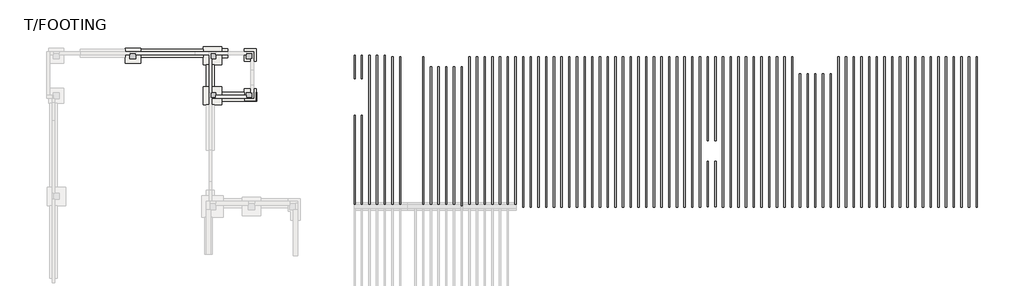
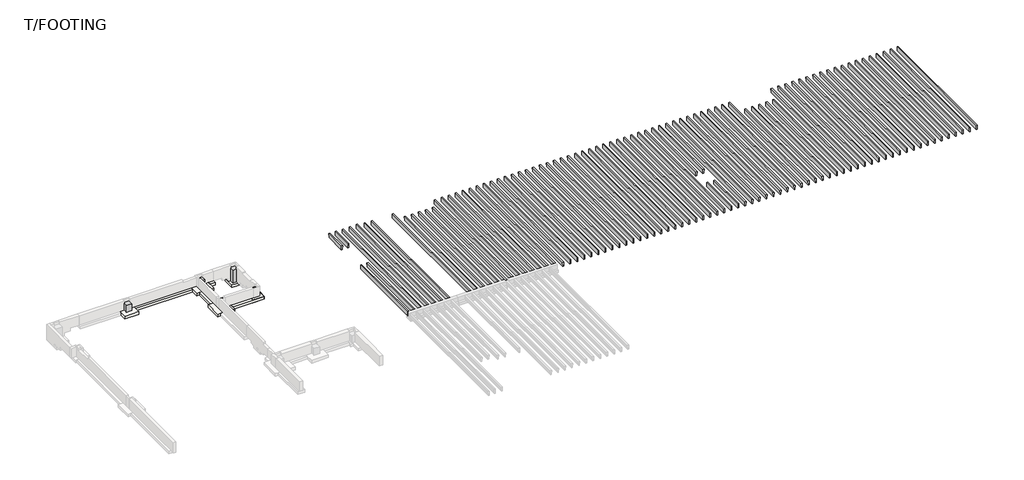
# One storey, part 3 of 3: 84 beams, 5 columns, 5 slabs, 4 footings.
# Revit data of these elements (continued)
# Elements 1, 2, 3, 4, 5, 6, 7, 8, 9, 10, 11, 12, 13, 14, 15, 16, 17, 18, 19, 20, 21, 22, 23, 24, 25, 26, 27, 28, 29, 30, 31, 32, 33, 34, 35, 36, 37, 38, 39, 40, 41, 42, 43, 44, 45, 46, 47, 48, 49, 50, 51, 52, 53, 54, 55, 56, 57, 58, 59, 60, 61, 62, 63, 82, 83, 84 (IfcBeam, "Precast-Cone Shaped Beam : DOUBLE_T") (continued)
#   Materials on its faces: "Concrete - Precast Concrete - Normal Weight Concrete - 5 ksi"
# Elements 64, 65 (IfcBeam, "Precast-Cone Shaped Beam : DOUBLE_T")
#   Comments = ""
#   Tie Rod Weight = 30
#   Tie Rod W = 0.0660938 kip
#   Single Rebar Weight = 50
#   Single Rebar W = 0.110156 kip
#   Rebar Grids Weight = 100
#   Rebar Grids W = 0.220313 kip
#   Length = 27' - 5 11/16"
#   Structural Material = Concrete - Precast Concrete - Normal Weight Concrete - 5 ksi
#   Phase Created = New Construction
#   Materials on its faces: "Concrete - Precast Concrete - Normal Weight Concrete - 5 ksi"
# Elements 66, 67 (IfcBeam, "Precast-Cone Shaped Beam : DOUBLE_T")
#   Comments = ""
#   Tie Rod Weight = 30
#   Tie Rod W = 0.0660938 kip
#   Single Rebar Weight = 50
#   Single Rebar W = 0.110156 kip
#   Rebar Grids Weight = 100
#   Rebar Grids W = 0.220313 kip
#   Length = 14' - 4 11/16"
#   Structural Material = Concrete - Precast Concrete - Normal Weight Concrete - 5 ksi
#   Phase Created = New Construction
#   Materials on its faces: "Concrete - Precast Concrete - Normal Weight Concrete - 5 ksi"
# Elements 68, 69, 70, 71, 72 (IfcBeam, "Precast-Cone Shaped Beam : DOUBLE_T")
#   Comments = ""
#   Tie Rod Weight = 30
#   Tie Rod W = 0.0660938 kip
#   Single Rebar Weight = 50
#   Single Rebar W = 0.110156 kip
#   Rebar Grids Weight = 100
#   Rebar Grids W = 0.220313 kip
#   Length = 42' - 9 11/16"
#   Structural Material = Concrete - Precast Concrete - Normal Weight Concrete - 5 ksi
#   Phase Created = New Construction
#   Materials on its faces: "Concrete - Precast Concrete - Normal Weight Concrete - 5 ksi"
# Elements 73, 74, 75, 76, 77 (IfcBeam, "Precast-Cone Shaped Beam : DOUBLE_T")
#   Comments = ""
#   Tie Rod Weight = 30
#   Tie Rod W = 0.0660938 kip
#   Single Rebar Weight = 50
#   Single Rebar W = 0.110156 kip
#   Rebar Grids Weight = 100
#   Rebar Grids W = 0.220313 kip
#   Length = 45' - 1 11/16"
#   Structural Material = Concrete - Precast Concrete - Normal Weight Concrete - 5 ksi
#   Phase Created = New Construction
#   Materials on its faces: "Concrete - Precast Concrete - Normal Weight Concrete - 5 ksi"
# Elements 78, 79 (IfcBeam, "Precast-Cone Shaped Beam : DOUBLE_T")
#   Comments = ""
#   Tie Rod Weight = 30
#   Tie Rod W = 0.0660938 kip
#   Single Rebar Weight = 50
#   Single Rebar W = 0.110156 kip
#   Rebar Grids Weight = 100
#   Rebar Grids W = 0.220313 kip
#   Length = 29' - 3.51269"
#   Structural Material = Concrete - Precast Concrete - Normal Weight Concrete - 5 ksi
#   Phase Created = New Construction
#   Materials on its faces: "Concrete - Precast Concrete - Normal Weight Concrete - 5 ksi"
# Elements 80, 81 (IfcBeam, "Precast-Cone Shaped Beam : DOUBLE_T")
#   Comments = ""
#   Tie Rod Weight = 30
#   Tie Rod W = 0.0660938 kip
#   Single Rebar Weight = 50
#   Single Rebar W = 0.110156 kip
#   Rebar Grids Weight = 100
#   Rebar Grids W = 0.220313 kip
#   Length = 7' - 4.11231"
#   Structural Material = Concrete - Precast Concrete - Normal Weight Concrete - 5 ksi
#   Phase Created = New Construction
#   Materials on its faces: "Concrete - Precast Concrete - Normal Weight Concrete - 5 ksi"
# Elements 85, 86 (IfcColumn, "Concrete-Square-Column : PIER 22\"x22\"")
#   Comments = ""
#   Structural Material = Concrete, Cast-in-Place gray
#   Phase Created = New Construction
#   Materials on its faces: "Concrete, Cast-in-Place gray"
# Elements 87, 88, 89 (IfcColumn, "Concrete-Square-Column : PIER 24\"x24\"")
#   Comments = ""
#   Structural Material = Concrete, Cast-in-Place gray
#   Phase Created = New Construction
#   Materials on its faces: "Concrete, Cast-in-Place gray"
# Elements 90, 91 (IfcFooting, "F4")
#   Phase Created = New Construction
#   Materials on its faces: "Concrete - Cast-in-Place Concrete"
# Elements 92, 93 (IfcFooting, "WF_30IN")
#   Phase Created = New Construction
#   Materials on its faces: "Default Floor"
# Elements 94, 95 (IfcSlab, "Spread Footing - Rectangular : F4")
#   Comments = ""
#   Phase Created = New Construction
#   Materials on its faces: "Concrete - Cast-in-Place Concrete"
# Element 96 (IfcSlab, "Spread Footing - Rectangular : F5")
#   Comments = ""
#   Structural Material = Concrete, Cast-in-Place gray
#   Phase Created = New Construction
#   Materials on its faces: "Concrete, Cast-in-Place gray"
# Elements 97, 98 (IfcSlab, "Spread Footing - Rectangular : F6")
#   Comments = ""
#   Structural Material = Concrete, Cast-in-Place gray
#   Phase Created = New Construction
#   Materials on its faces: "Concrete, Cast-in-Place gray"
# Materials
#   "Concrete, Precast": class "Concrete", colour RGB 198 187 187, transparency 0, Description = "Precast concrete", Cost = 0
#   "Concrete, Cast-in-Place gray": class "Concrete", colour RGB 192 192 192, transparency 0, Description = "Cast-in-place concrete", Cost = 0
#   "Concrete - Cast-in-Place Concrete": class "Concrete", colour RGB 192 192 192, transparency 0, Description = "Concrete", Cost = 0
#   "Concrete - Precast Concrete - Normal Weight Concrete - 5 ksi": class "Concrete", colour RGB 198 187 187, transparency 0, Cost = 0
#   "Default Floor": class "Miscellaneous", colour RGB 128 128 128, transparency 0, Cost = 0
